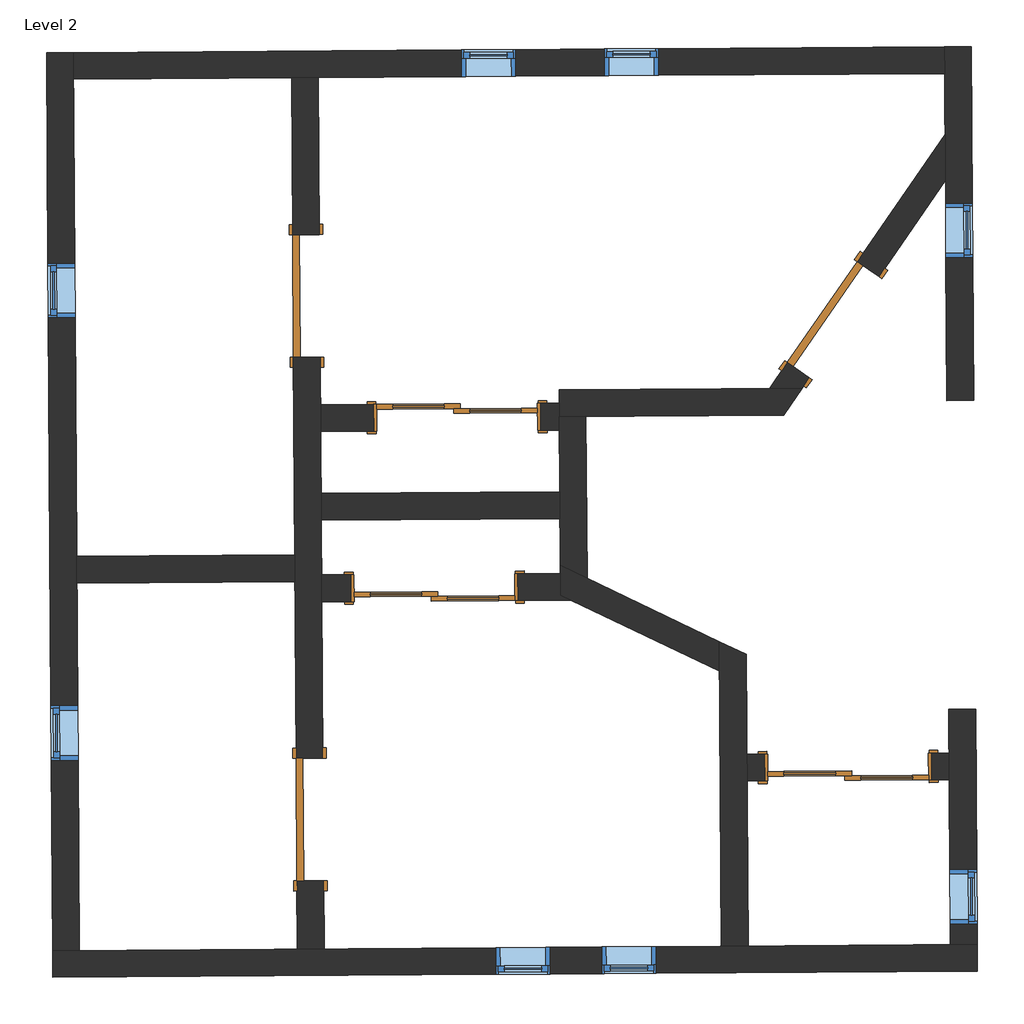
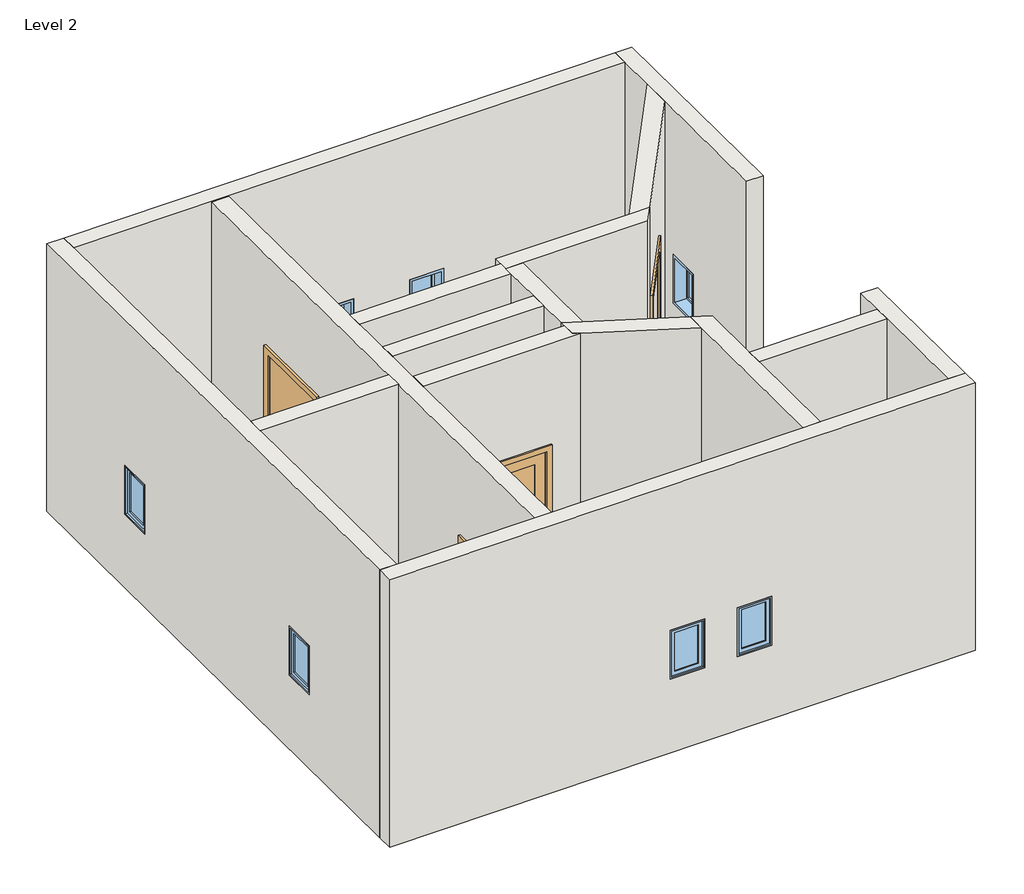
# One storey: 16 walls, 8 windows, 6 doors.
"""IFC4 building model written with IfcOpenShell, lengths in millimetres."""

import ifcopenshell
import ifcopenshell.guid

model = None  # the IFC model being written
_history = None  # IfcOwnerHistory: only IFC2X3 demands one
_inside = {}  # id of a spatial element -> (the spatial element, [elements in it])
_under = {}  # id of a project, library or spatial element -> (it, [spatial elements below it])
_declared = {}  # id of a project -> (the project, [libraries it declares])
_typed = {}  # id of a type object -> (the type object, [elements of that type])
_made_of = {}  # id of a material, layer set ... -> (it, [elements and type objects made of it])


def new_model(schema):
    """Start an empty IFC model of exactly this schema.

    Asked for "IFC4X3", IfcOpenShell would pick the latest addendum, in which some entities
    have other attributes; the version numbers below select the first issue.
    IFC2X3 requires an IfcOwnerHistory on every rooted entity: one is made here for all.
    """
    global model, _history
    if schema == "IFC4X3":
        model = ifcopenshell.file(schema_version=(4, 3, 0, 0))
    else:
        model = ifcopenshell.file(schema=schema)
    _inside.clear()
    _under.clear()
    _declared.clear()
    _typed.clear()
    _made_of.clear()
    _history = None
    if model.schema == "IFC2X3":
        org = make("IfcOrganization", Name="unknown")
        user = make(
            "IfcPersonAndOrganization",
            ThePerson=make("IfcPerson", FamilyName="unknown"),
            TheOrganization=org,
        )
        app = make(
            "IfcApplication",
            ApplicationDeveloper=org,
            Version="unknown",
            ApplicationFullName="unknown",
            ApplicationIdentifier="unknown",
        )
        _history = make(
            "IfcOwnerHistory",
            OwningUser=user,
            OwningApplication=app,
            ChangeAction="ADDED",
            CreationDate=0,
        )
    return model


def make(cls, **values):
    """One entity of the class cls with the attributes given. An attribute that is None is left unset."""
    return model.create_entity(
        cls, **{name: value for name, value in values.items() if value is not None}
    )


def rooted(cls, **values):
    """An entity with a GlobalId (a new one), such as an element, a storey or a relation."""
    return make(cls, GlobalId=ifcopenshell.guid.new(), OwnerHistory=_history, **values)


def si_unit(unit_type, name, prefix=None):
    """IfcSIUnit, for example si_unit("LENGTHUNIT", "METRE", prefix="MILLI")."""
    return make("IfcSIUnit", UnitType=unit_type, Prefix=prefix, Name=name)


def assignment(units):
    """IfcUnitAssignment: the units of a project."""
    return None if units is None else make("IfcUnitAssignment", Units=units)


def point(xyz):
    """IfcCartesianPoint."""
    return None if xyz is None else make("IfcCartesianPoint", Coordinates=xyz)


def direction(xyz):
    """IfcDirection."""
    return None if xyz is None else make("IfcDirection", DirectionRatios=xyz)


def frame(location, z_axis=None, x_axis=None):
    """IfcAxis2Placement3D, a coordinate frame: its origin and axes. An axis left out is left unset."""
    return make(
        "IfcAxis2Placement3D",
        Location=point(location),
        Axis=direction(z_axis),
        RefDirection=direction(x_axis),
    )


def origin():
    """The frame at (0, 0, 0) with its axes left unset."""
    return frame((0.0, 0.0, 0.0))


def origin_with_axes():
    """The frame at (0, 0, 0) with the z axis (0, 0, 1) and the x axis (1, 0, 0) written out."""
    return frame((0.0, 0.0, 0.0), z_axis=(0.0, 0.0, 1.0), x_axis=(1.0, 0.0, 0.0))


def place(relative_to, where):
    """IfcLocalPlacement: puts the frame where relative to a parent placement (None: the world)."""
    return make(
        "IfcLocalPlacement", PlacementRelTo=relative_to, RelativePlacement=where
    )


def context(
    kind, dimensions, precision=None, world=None, true_north=None, identifier=None
):
    """IfcGeometricRepresentationContext, for example the 3D "Model" context."""
    return make(
        "IfcGeometricRepresentationContext",
        ContextIdentifier=identifier,
        ContextType=kind,
        CoordinateSpaceDimension=dimensions,
        Precision=precision,
        WorldCoordinateSystem=world,
        TrueNorth=true_north,
    )


def project(units=None, contexts=None):
    """IfcProject with its units and contexts."""
    return rooted(
        "IfcProject",
        Name="project",
        RepresentationContexts=contexts,
        UnitsInContext=assignment(units),
    )


def spatial(cls, under=None, at=None, **own):
    """A site, building, storey or space (cls), placed at a placement, below another one or the project."""
    s = rooted(cls, ObjectPlacement=at, **own)
    if under is not None:
        _under.setdefault(under.id(), (under, []))[1].append(s)
    return s


def polyline(points):
    """IfcPolyline through the points."""
    return make("IfcPolyline", Points=[point(p) for p in points])


def outline(outer, holes=None, kind="AREA"):
    """IfcArbitraryClosedProfileDef: a profile drawn as a closed curve; with holes, ...WithVoids."""
    if holes is None:
        return make("IfcArbitraryClosedProfileDef", ProfileType=kind, OuterCurve=outer)
    return make(
        "IfcArbitraryProfileDefWithVoids",
        ProfileType=kind,
        OuterCurve=outer,
        InnerCurves=holes,
    )


def extrude(swept, where, along, depth):
    """IfcExtrudedAreaSolid: the profile swept, set in the frame where, extruded along a direction by depth."""
    return make(
        "IfcExtrudedAreaSolid",
        SweptArea=swept,
        Position=where,
        ExtrudedDirection=direction(along),
        Depth=depth,
    )


def faces_of(points, faces, orient=None, outer=None):
    """IfcFace entities. A face is a list of loops; a loop is a list of indices into points, from 0.

    orient and outer hold one flag for each loop. By default every Orientation is true, the
    first loop of a face is its IfcFaceOuterBound and the others are IfcFaceBound.
    """
    made = []
    for i, loops in enumerate(faces):
        bounds = []
        for j, loop in enumerate(loops):
            is_outer = j == 0 if outer is None else outer[i][j]
            bounds.append(
                make(
                    "IfcFaceOuterBound" if is_outer else "IfcFaceBound",
                    Bound=make("IfcPolyLoop", Polygon=[points[k] for k in loop]),
                    Orientation=True if orient is None else orient[i][j],
                )
            )
        made.append(make("IfcFace", Bounds=bounds))
    return made


def faceted_brep(points, faces, orient=None, outer=None, voids=None):
    """IfcFacetedBrep: a solid bounded by flat faces; with voids (closed shells), ...WithVoids."""
    shared = [point(p) for p in points]
    hull = make("IfcClosedShell", CfsFaces=faces_of(shared, faces, orient, outer))
    if voids is None:
        return make("IfcFacetedBrep", Outer=hull)
    return make(
        "IfcFacetedBrepWithVoids",
        Outer=hull,
        Voids=[
            make(cls, CfsFaces=faces_of(shared, fs, o, b)) for cls, fs, o, b in voids
        ],
    )


def shape(context_of_items, identifier, shape_type, items):
    """IfcShapeRepresentation: the items that make up one representation, for example the "Body"."""
    return make(
        "IfcShapeRepresentation",
        ContextOfItems=context_of_items,
        RepresentationIdentifier=identifier,
        RepresentationType=shape_type,
        Items=items,
    )


def source(mapping_origin, context_of_items, identifier, shape_type, items):
    """IfcRepresentationMap: a shape defined once, which mapped items show again and again."""
    return make(
        "IfcRepresentationMap",
        MappingOrigin=mapping_origin,
        MappedRepresentation=shape(context_of_items, identifier, shape_type, items),
    )


def transform(
    local_origin,
    x_axis=None,
    y_axis=None,
    z_axis=None,
    scale=None,
    scale2=None,
    scale3=None,
    uniform=True,
):
    """IfcCartesianTransformationOperator3D, or its non-uniform kind. x_axis, y_axis, z_axis: its Axis1, 2, 3."""
    if uniform:
        return make(
            "IfcCartesianTransformationOperator3D",
            Axis1=direction(x_axis),
            Axis2=direction(y_axis),
            LocalOrigin=point(local_origin),
            Scale=scale,
            Axis3=direction(z_axis),
        )
    return make(
        "IfcCartesianTransformationOperator3DnonUniform",
        Axis1=direction(x_axis),
        Axis2=direction(y_axis),
        LocalOrigin=point(local_origin),
        Scale=scale,
        Axis3=direction(z_axis),
        Scale2=scale2,
        Scale3=scale3,
    )


def mapped(mapping_source, mapping_target):
    """IfcMappedItem: shows the shape of a source again, moved by a transform."""
    return make(
        "IfcMappedItem", MappingSource=mapping_source, MappingTarget=mapping_target
    )


def made_of(thing, what):
    """Note that an element or type object is made of a material, layer set ...; save() writes the relation."""
    if what is not None:
        _made_of.setdefault(what.id(), (what, []))[1].append(thing)
    return thing


def element(
    cls,
    number,
    at=None,
    inside=None,
    cuts=None,
    type_object=None,
    material=None,
    context=None,
    identifier="Body",
    shape_type=None,
    held_by="IfcProductDefinitionShape",
    body=None,
    shapes=None,
    **own,
):
    """One element of the class cls, such as IfcWall. Its Tag is "e" and its number.

    at: its placement. inside: the storey or other place that contains it. cuts: it is an
    opening in that element (IfcRelVoidsElement). A single representation is given by context,
    identifier, shape_type and body (its items); several are given by shapes. held_by: the class
    of the entity that holds the representations. save() writes the other relations.
    """
    e = rooted(cls, Tag="e%d" % number, ObjectPlacement=at, **own)
    if body is not None:
        shapes = [shape(context, identifier, shape_type, body)]
    if shapes is not None:
        e.Representation = make(held_by, Representations=shapes)
    if inside is not None:
        _inside.setdefault(inside.id(), (inside, []))[1].append(e)
    if cuts is not None:
        rooted(
            "IfcRelVoidsElement", RelatingBuildingElement=cuts, RelatedOpeningElement=e
        )
    if type_object is not None:
        _typed.setdefault(type_object.id(), (type_object, []))[1].append(e)
    return made_of(e, material)


def aggregate(whole, parts):
    """IfcRelAggregates: a whole, such as a stair, and the parts it consists of."""
    return rooted("IfcRelAggregates", RelatingObject=whole, RelatedObjects=parts)


def save(model, path):
    """Write the relations noted so far, then the file.

    IfcRelAggregates (storeys below a building ...), IfcRelContainedInSpatialStructure (elements
    in a storey), IfcRelDefinesByType, IfcRelAssociatesMaterial and IfcRelDeclares: one each for
    every whole, place, type object, material and project.
    """
    for whole, parts in _under.values():
        aggregate(whole, parts)
    for where, things in _inside.values():
        rooted(
            "IfcRelContainedInSpatialStructure",
            RelatedElements=things,
            RelatingStructure=where,
        )
    for kind, things in _typed.values():
        rooted("IfcRelDefinesByType", RelatedObjects=things, RelatingType=kind)
    for what, things in _made_of.values():
        rooted("IfcRelAssociatesMaterial", RelatedObjects=things, RelatingMaterial=what)
    for by, libraries in _declared.values():
        rooted("IfcRelDeclares", RelatingContext=by, RelatedDefinitions=libraries)
    model.write(path)


def m_door_interior_double_sliding_2_panel_wood_1200_x_2000mm_2523b4d6(model_context):
    return source(origin(), model_context, "Body", "SweptSolid", [
        extrude(outline(polyline([(480.0, 38.4916667), (94.6, 38.4916667), (94.6, 50.1583333), (480.0, 50.1583333), (480.0, 38.4916667)])), frame((0.0, 0.0, 1014.4), z_axis=(0.0, 0.0, 1.0), x_axis=(1.0, 0.0, 0.0)), (0.0, 0.0, 1.0), 865.6),
        extrude(outline(polyline([(480.0, 38.4916667), (94.6, 38.4916667), (94.6, 50.1583333), (480.0, 50.1583333), (480.0, 38.4916667)])), frame((0.0, 0.0, 230.0), z_axis=(0.0, 0.0, 1.0), x_axis=(1.0, 0.0, 0.0)), (0.0, 0.0, 1.0), 584.4),
        extrude(outline(polyline([(2000.0, -25.4), (0.0, -25.4), (0.0, 600.0), (2000.0, 600.0), (2000.0, -25.4)]), holes=[polyline([(1880.0, 94.6), (1880.0, 480.0), (1014.4, 480.0), (1014.4, 94.6), (1880.0, 94.6)]), polyline([(814.4, 94.6), (814.4, 480.0), (230.0, 480.0), (230.0, 94.6), (814.4, 94.6)])]), frame((0.0, 26.825, 0.0), z_axis=(0.0, 1.0, 0.0), x_axis=(0.0, 0.0, 1.0)), (0.0, 0.0, 1.0), 35.0),
        extrude(outline(polyline([(-94.6, 73.4916667), (-480.0, 73.4916667), (-480.0, 85.1583333), (-94.6, 85.1583333), (-94.6, 73.4916667)])), frame((0.0, 0.0, 1014.4), z_axis=(0.0, 0.0, 1.0), x_axis=(1.0, 0.0, 0.0)), (0.0, 0.0, 1.0), 865.6),
        extrude(outline(polyline([(-94.6, 73.4916667), (-480.0, 73.4916667), (-480.0, 85.1583333), (-94.6, 85.1583333), (-94.6, 73.4916667)])), frame((0.0, 0.0, 230.0), z_axis=(0.0, 0.0, 1.0), x_axis=(1.0, 0.0, 0.0)), (0.0, 0.0, 1.0), 584.4),
        extrude(outline(polyline([(2000.0, -600.0), (0.0, -600.0), (0.0, 25.4), (2000.0, 25.4), (2000.0, -600.0)]), holes=[polyline([(1880.0, -480.0), (1880.0, -94.6), (1014.4, -94.6), (1014.4, -480.0), (1880.0, -480.0)]), polyline([(814.4, -480.0), (814.4, -94.6), (230.0, -94.6), (230.0, -480.0), (814.4, -480.0)])]), frame((0.0, 61.825, 0.0), z_axis=(0.0, 1.0, 0.0), x_axis=(0.0, 0.0, 1.0)), (0.0, 0.0, 1.0), 35.0),
        extrude(outline(polyline([(0.0, 600.0), (0.0, 625.0), (2025.0, 625.0), (2025.0, -625.0), (0.0, -625.0), (0.0, -600.0), (2000.0, -600.0), (2000.0, 600.0), (0.0, 600.0)])), frame((0.0, -103.175, 0.0), z_axis=(0.0, 1.0, 0.0), x_axis=(0.0, 0.0, 1.0)), (0.0, 0.0, 1.0), 200.0),
        extrude(outline(polyline([(0.0, 606.35), (0.0, 671.35), (2071.35, 671.35), (2071.35, -671.35), (0.0, -671.35), (0.0, -606.35), (2006.35, -606.35), (2006.35, 606.35), (0.0, 606.35)])), frame((0.0, -123.175, 0.0), z_axis=(0.0, 1.0, 0.0), x_axis=(0.0, 0.0, 1.0)), (0.0, 0.0, 1.0), 20.0),
        extrude(outline(polyline([(0.0, 606.35), (0.0, 671.35), (2071.35, 671.35), (2071.35, -671.35), (0.0, -671.35), (0.0, -606.35), (2006.35, -606.35), (2006.35, 606.35), (0.0, 606.35)])), frame((0.0, 96.825, 0.0), z_axis=(0.0, 1.0, 0.0), x_axis=(0.0, 0.0, 1.0)), (0.0, 0.0, 1.0), 20.0),
    ])


def m_single_flush_0915_x_2134mm_6a9e8738(model_context):
    return source(origin(), model_context, "Body", "SweptSolid", [
        extrude(outline(polyline([(2210.0, -533.5), (0.0, -533.5), (0.0, -457.5), (2134.0, -457.5), (2134.0, 457.5), (0.0, 457.5), (0.0, 533.5), (2210.0, 533.5), (2210.0, -533.5)])), frame((0.0, 100.0, 0.0), z_axis=(0.0, 1.0, 0.0), x_axis=(0.0, 0.0, 1.0)), (0.0, 0.0, 1.0), 25.0),
        extrude(outline(polyline([(2210.0, 533.5), (2210.0, -533.5), (0.0, -533.5), (0.0, -457.5), (2134.0, -457.5), (2134.0, 457.5), (0.0, 457.5), (0.0, 533.5), (2210.0, 533.5)])), frame((0.0, -125.0, 0.0), z_axis=(0.0, 1.0, 0.0), x_axis=(0.0, 0.0, 1.0)), (0.0, 0.0, 1.0), 25.0),
        extrude(outline(polyline([(457.5, 49.0), (-457.5, 49.0), (-457.5, 100.0), (457.5, 100.0), (457.5, 49.0)])), origin_with_axes(), (0.0, 0.0, 1.0), 2134.0),
    ])


def m_single_flush_0915_x_2134mm_727434cd(model_context):
    return source(origin(), model_context, "Body", "SweptSolid", [
        extrude(outline(polyline([(2210.0, -533.5), (0.0, -533.5), (0.0, -457.5), (2134.0, -457.5), (2134.0, 457.5), (0.0, 457.5), (0.0, 533.5), (2210.0, 533.5), (2210.0, -533.5)])), frame((0.0, -125.0, 0.0), z_axis=(0.0, 1.0, 0.0), x_axis=(0.0, 0.0, 1.0)), (0.0, 0.0, 1.0), 25.0),
        extrude(outline(polyline([(2210.0, 533.5), (2210.0, -533.5), (0.0, -533.5), (0.0, -457.5), (2134.0, -457.5), (2134.0, 457.5), (0.0, 457.5), (0.0, 533.5), (2210.0, 533.5)])), frame((0.0, 100.0, 0.0), z_axis=(0.0, 1.0, 0.0), x_axis=(0.0, 0.0, 1.0)), (0.0, 0.0, 1.0), 25.0),
        extrude(outline(polyline([(457.5, -49.0), (457.5, -100.0), (-457.5, -100.0), (-457.5, -49.0), (457.5, -49.0)])), origin_with_axes(), (0.0, 0.0, 1.0), 2134.0),
    ])


def m_fixed_0406_x_0610mm_8205b201(model_context):
    return source(origin(), model_context, "Body", "SweptSolid", [
        extrude(outline(polyline([(-140.0, 78.0), (140.0, 78.0), (140.0, 66.0), (-140.0, 66.0), (-140.0, 78.0)])), frame((0.0, 0.0, 978.0), z_axis=(0.0, 0.0, 1.0), x_axis=(1.0, 0.0, 0.0)), (0.0, 0.0, 1.0), 484.0),
        extrude(outline(polyline([(1506.0, -184.0), (934.0, -184.0), (934.0, 184.0), (1506.0, 184.0), (1506.0, -184.0)]), holes=[polyline([(1462.0, -140.0), (1462.0, 140.0), (978.0, 140.0), (978.0, -140.0), (1462.0, -140.0)])]), frame((0.0, 50.0, 0.0), z_axis=(0.0, 1.0, 0.0), x_axis=(0.0, 0.0, 1.0)), (0.0, 0.0, 1.0), 44.0),
        extrude(outline(polyline([(1525.0, -203.0), (915.0, -203.0), (915.0, 203.0), (1525.0, 203.0), (1525.0, -203.0)]), holes=[polyline([(1506.0, -184.0), (1506.0, 184.0), (934.0, 184.0), (934.0, -184.0), (1506.0, -184.0)])]), frame((0.0, 50.0, 0.0), z_axis=(0.0, 1.0, 0.0), x_axis=(0.0, 0.0, 1.0)), (0.0, 0.0, 1.0), 63.0),
        extrude(outline(polyline([(1525.0, -203.0), (915.0, -203.0), (915.0, 203.0), (1525.0, 203.0), (1525.0, -203.0)]), holes=[polyline([(1493.0, -171.0), (1493.0, 171.0), (947.0, 171.0), (947.0, -171.0), (1493.0, -171.0)])]), frame((0.0, -87.0, 0.0), z_axis=(0.0, 1.0, 0.0), x_axis=(0.0, 0.0, 1.0)), (0.0, 0.0, 1.0), 137.0),
    ])


model = new_model("IFC4")

# Units and contexts
model_context = context("Model", 3, world=origin())
ifc_project = project(units=[si_unit("LENGTHUNIT", "METRE", prefix="MILLI")], contexts=[model_context])

# Site, building, storey
site = spatial("IfcSite", under=ifc_project)
building = spatial("IfcBuilding", under=site)
storey = spatial("IfcBuildingStorey", under=building, Name="Level 2", Elevation=3048.0)

# Doors
placement = place(None, origin())
m_door_interior_double_sliding_2_panel_wood_1200_x_2000mm_shape = m_door_interior_double_sliding_2_panel_wood_1200_x_2000mm_2523b4d6(model_context)
element("IfcDoor", 1, ObjectType="M_Door-Interior-Double-Sliding-2_Panel-Wood : 1200 x 2000mm", at=placement, inside=storey, context=model_context, shape_type="MappedRepresentation", body=[
    mapped(m_door_interior_double_sliding_2_panel_wood_1200_x_2000mm_shape, transform((-90488.9924739, -37950.707077, 3048.0), x_axis=(0.9999777944135733, 0.006664133834601911, 0.0), y_axis=(-0.006664133834601911, 0.9999777944135733, 0.0), z_axis=(0.0, 0.0, 1.0))),
])
element("IfcDoor", 2, ObjectType="M_Door-Interior-Double-Sliding-2_Panel-Wood : 1200 x 2000mm", at=placement, inside=storey, context=model_context, shape_type="MappedRepresentation", body=[
    mapped(m_door_interior_double_sliding_2_panel_wood_1200_x_2000mm_shape, transform((-90659.0777486, -39228.968042, 3048.0), x_axis=(-0.9999777944135733, -0.006664133834601911, 0.0), y_axis=(0.006664133834601911, -0.9999777944135733, 0.0), z_axis=(0.0, 0.0, 1.0))),
])
element("IfcDoor", 3, ObjectType="M_Door-Interior-Double-Sliding-2_Panel-Wood : 1200 x 2000mm", at=placement, inside=storey, context=model_context, shape_type="MappedRepresentation", body=[
    mapped(m_door_interior_double_sliding_2_panel_wood_1200_x_2000mm_shape, transform((-87568.9864205, -40568.3479238, 3048.0), x_axis=(-0.9999777944135733, -0.006664133834601911, 0.0), y_axis=(0.006664133834601911, -0.9999777944135733, 0.0), z_axis=(0.0, 0.0, 1.0))),
])
m_single_flush_0915_x_2134mm_shape = m_single_flush_0915_x_2134mm_6a9e8738(model_context)
element("IfcDoor", 4, ObjectType="M_Single-Flush : 0915 x 2134mm", at=placement, inside=storey, context=model_context, shape_type="MappedRepresentation", body=[
    mapped(m_single_flush_0915_x_2134mm_shape, transform((-87680.4573367, -37224.8879698, 3048.0), x_axis=(0.5681047608958888, 0.8229562446736918, 0.0), y_axis=(-0.8229562446736918, 0.5681047608958888, 0.0), z_axis=(0.0, 0.0, 1.0))),
])
element("IfcDoor", 5, ObjectType="M_Single-Flush : 0915 x 2134mm", at=placement, inside=storey, context=model_context, shape_type="MappedRepresentation", body=[
    mapped(m_single_flush_0915_x_2134mm_shape, transform((-91614.2394972, -37047.0582792, 3048.0), x_axis=(-0.0066641338345986775, 0.9999777944135734, 0.0), y_axis=(-0.9999777944135734, -0.0066641338345986775, 0.0), z_axis=(0.0, 0.0, 1.0))),
])
m_single_flush_0915_x_2134mm_2_shape = m_single_flush_0915_x_2134mm_727434cd(model_context)
element("IfcDoor", 6, ObjectType="M_Single-Flush : 0915 x 2134mm", at=placement, inside=storey, context=model_context, shape_type="MappedRepresentation", body=[
    mapped(m_single_flush_0915_x_2134mm_2_shape, transform((-91588.1820843, -40957.0689247, 3048.0), x_axis=(0.0066641338345986775, -0.9999777944135734, 0.0), y_axis=(0.9999777944135734, 0.0066641338345986775, 0.0), z_axis=(0.0, 0.0, 1.0))),
])

# Walls
element("IfcWall", 7, ObjectType="Generic - 200mm", at=placement, inside=storey, context=model_context, shape_type="Brep", body=[
    faceted_brep([(-86605.0497125, -41890.681395, 3048.0), (-86805.0452714, -41892.0142218, 3048.0), (-88315.2179284, -41902.078438, 3048.0), (-88515.2134873, -41903.4112648, 3048.0), (-91481.7414203, -41923.1810429, 3048.0), (-91681.7369792, -41924.5138697, 3048.0), (-93310.5008107, -41935.3684109, 3048.0), (-93510.4963696, -41936.7012377, 3048.0), (-93510.4963696, -41936.7012377, 6372.225), (-93310.5008107, -41935.3684109, 6372.225), (-88515.2134873, -41903.4112648, 6372.225), (-88315.2179284, -41902.078438, 6372.225), (-86805.0452714, -41892.0142218, 6372.225), (-86605.0497125, -41890.681395, 6372.225), (-89795.4819615, -41911.9433347, 3963.0), (-89795.4819615, -41911.9433347, 4573.0), (-90201.4729461, -41914.648973, 4573.0), (-90201.4729461, -41914.648973, 3963.0), (-89003.8510886, -41906.6676834, 3963.0), (-89003.8510886, -41906.6676834, 4573.0), (-89409.8420731, -41909.3733218, 4573.0), (-89409.8420731, -41909.3733218, 3963.0), (-86603.7168857, -42090.6769539, 3048.0), (-86603.7168857, -42090.6769539, 6372.225), (-93509.1635428, -42136.6967965, 6372.225), (-93509.1635428, -42136.6967965, 3048.0), (-89794.1491348, -42111.9388936, 3963.0), (-90200.1401193, -42114.6445319, 3963.0), (-90200.1401193, -42114.6445319, 4573.0), (-89794.1491348, -42111.9388936, 4573.0), (-89002.5182618, -42106.6632423, 3963.0), (-89408.5092463, -42109.3688807, 3963.0), (-89408.5092463, -42109.3688807, 4573.0), (-89002.5182618, -42106.6632423, 4573.0)], [[[0, 1, 2, 3, 4, 5, 6, 7, 8, 9, 10, 11, 12, 13], [14, 15, 16, 17], [18, 19, 20, 21]], [[22, 23, 24, 25], [26, 27, 28, 29], [30, 31, 32, 33]], [[8, 7, 25, 24]], [[0, 13, 23, 22]], [[15, 14, 26, 29]], [[16, 15, 29, 28]], [[17, 16, 28, 27]], [[14, 17, 27, 26]], [[19, 18, 30, 33]], [[20, 19, 33, 32]], [[21, 20, 32, 31]], [[18, 21, 31, 30]], [[7, 6, 5, 4, 3, 2, 1, 0, 22, 25]], [[13, 12, 11, 10, 9, 8, 24, 23]]]),
])
element("IfcWall", 8, ObjectType="Generic - 200mm", at=placement, inside=storey, context=model_context, shape_type="Brep", body=[
    faceted_brep([(-93310.5008107, -41935.3684109, 3048.0), (-93328.7831618, -39192.0343866, 3048.0), (-93330.1159886, -38992.0388277, 3048.0), (-93353.8549998, -35429.9128716, 3048.0), (-93355.1878266, -35229.9173127, 3048.0), (-93355.1878266, -35229.9173127, 6372.225), (-93353.8549998, -35429.9128716, 6372.225), (-93330.1159886, -38992.0388277, 6372.225), (-93328.7831618, -39192.0343866, 6372.225), (-93310.5008107, -41935.3684109, 6372.225), (-93341.9968401, -37209.2733589, 3963.0), (-93341.9968401, -37209.2733589, 4573.0), (-93344.7024784, -36803.2823744, 4573.0), (-93344.7024784, -36803.2823744, 3963.0), (-93319.971844, -40514.2050264, 3963.0), (-93319.971844, -40514.2050264, 4573.0), (-93322.6774824, -40108.2140418, 4573.0), (-93322.6774824, -40108.2140418, 3963.0), (-93510.4963696, -41936.7012377, 3048.0), (-93510.4963696, -41936.7012377, 6372.225), (-93555.1833855, -35231.2501394, 6372.225), (-93555.1833855, -35231.2501394, 3048.0), (-93541.9923989, -37210.6061857, 3963.0), (-93544.6980373, -36804.6152012, 3963.0), (-93544.6980373, -36804.6152012, 4573.0), (-93541.9923989, -37210.6061857, 4573.0), (-93519.9674029, -40515.5378531, 3963.0), (-93522.6730413, -40109.5468686, 3963.0), (-93522.6730413, -40109.5468686, 4573.0), (-93519.9674029, -40515.5378531, 4573.0)], [[[0, 1, 2, 3, 4, 5, 6, 7, 8, 9], [10, 11, 12, 13], [14, 15, 16, 17]], [[18, 19, 20, 21], [22, 23, 24, 25], [26, 27, 28, 29]], [[4, 3, 2, 1, 0, 18, 21]], [[9, 8, 7, 6, 5, 20, 19]], [[0, 9, 19, 18]], [[5, 4, 21, 20]], [[11, 10, 22, 25]], [[12, 11, 25, 24]], [[13, 12, 24, 23]], [[10, 13, 23, 22]], [[15, 14, 26, 29]], [[16, 15, 29, 28]], [[17, 16, 28, 27]], [[14, 17, 27, 26]]]),
])
element("IfcWall", 9, ObjectType="Generic - 200mm", at=placement, inside=storey, context=model_context, shape_type="Brep", body=[
    faceted_brep([(-93353.8549998, -35429.9128716, 3048.0), (-91725.0911683, -35419.0583304, 3048.0), (-91525.0956094, -35417.7255036, 3048.0), (-86848.3994605, -35386.5586825, 3048.0), (-86848.3994605, -35386.5586825, 6372.225), (-93353.8549998, -35429.9128716, 6372.225), (-89389.7430272, -35403.4949122, 3963.0), (-89389.7430272, -35403.4949122, 4573.0), (-88983.7520427, -35400.7892739, 4573.0), (-88983.7520427, -35400.7892739, 3963.0), (-90456.5193383, -35410.6042102, 3963.0), (-90456.5193383, -35410.6042102, 4573.0), (-90050.5283537, -35407.8985718, 4573.0), (-90050.5283537, -35407.8985718, 3963.0), (-93355.1878266, -35229.9173127, 3048.0), (-93355.1878266, -35229.9173127, 6372.225), (-86849.7322872, -35186.5631236, 6372.225), (-86849.7322872, -35186.5631236, 3048.0), (-89391.075854, -35203.4993533, 3963.0), (-88985.0848694, -35200.793715, 3963.0), (-88985.0848694, -35200.793715, 4573.0), (-89391.075854, -35203.4993533, 4573.0), (-90457.852165, -35210.6086513, 3963.0), (-90051.8611805, -35207.903013, 3963.0), (-90051.8611805, -35207.903013, 4573.0), (-90457.852165, -35210.6086513, 4573.0)], [[[0, 1, 2, 3, 4, 5], [6, 7, 8, 9], [10, 11, 12, 13]], [[14, 15, 16, 17], [18, 19, 20, 21], [22, 23, 24, 25]], [[3, 2, 1, 0, 14, 17]], [[5, 4, 16, 15]], [[0, 5, 15, 14]], [[7, 6, 18, 21]], [[8, 7, 21, 20]], [[9, 8, 20, 19]], [[6, 9, 19, 18]], [[11, 10, 22, 25]], [[12, 11, 25, 24]], [[13, 12, 24, 23]], [[10, 13, 23, 22]], [[4, 3, 17, 16]]]),
])
element("IfcWall", 10, ObjectType="Generic - 200mm", at=placement, inside=storey, context=model_context, shape_type="Brep", body=[
    faceted_brep([(-86849.7322872, -35186.5631236, 3048.0), (-86848.3994605, -35386.5586825, 3048.0), (-86845.3830911, -35839.1760037, 3048.0), (-86843.0593785, -36187.85762, 3048.0), (-86832.1189478, -37829.5094911, 3048.0), (-86832.1189478, -37829.5094911, 6372.225), (-86843.0593785, -36187.85762, 6372.225), (-86845.3830911, -35839.1760037, 6372.225), (-86848.3994605, -35386.5586825, 6372.225), (-86849.7322872, -35186.5631236, 6372.225), (-86841.94523, -36355.0397048, 3963.0), (-86841.94523, -36355.0397048, 4573.0), (-86839.2395917, -36761.0306894, 4573.0), (-86839.2395917, -36761.0306894, 3963.0), (-86649.7367284, -35185.2302968, 3048.0), (-86649.7367284, -35185.2302968, 6372.225), (-86632.1233889, -37828.1766644, 6372.225), (-86632.1233889, -37828.1766644, 3048.0), (-86641.9496711, -36353.7068781, 3963.0), (-86639.2440328, -36759.6978626, 3963.0), (-86639.2440328, -36759.6978626, 4573.0), (-86641.9496711, -36353.7068781, 4573.0)], [[[0, 1, 2, 3, 4, 5, 6, 7, 8, 9], [10, 11, 12, 13]], [[14, 15, 16, 17], [18, 19, 20, 21]], [[4, 3, 2, 1, 0, 14, 17]], [[5, 4, 17, 16]], [[9, 8, 7, 6, 5, 16, 15]], [[11, 10, 18, 21]], [[12, 11, 21, 20]], [[13, 12, 20, 19]], [[10, 13, 19, 18]], [[0, 9, 15, 14]]]),
])
element("IfcWall", 11, ObjectType="Generic - 200mm", at=placement, inside=storey, context=model_context, shape_type="Brep", body=[
    faceted_brep([(-86605.0497125, -41890.681395, 3048.0), (-86616.7572548, -40133.9216051, 3048.0), (-86616.7572548, -40133.9216051, 6372.225), (-86605.0497125, -41890.681395, 6372.225), (-86608.7829603, -41330.4938346, 3963.0), (-86606.077322, -41736.4848191, 3963.0), (-86606.077322, -41736.4848191, 4573.0), (-86608.7829603, -41330.4938346, 4573.0), (-86805.0452714, -41892.0142218, 3048.0), (-86805.0452714, -41892.0142218, 6372.225), (-86813.2548373, -40660.1386656, 6372.225), (-86814.587664, -40460.1431068, 6372.225), (-86816.7528137, -40135.2544319, 6372.225), (-86816.7528137, -40135.2544319, 3048.0), (-86814.587664, -40460.1431068, 3048.0), (-86813.2548373, -40660.1386656, 3048.0), (-86808.7785192, -41331.8266614, 3963.0), (-86808.7785192, -41331.8266614, 4573.0), (-86806.0728808, -41737.8176459, 4573.0), (-86806.0728808, -41737.8176459, 3963.0)], [[[0, 1, 2, 3], [4, 5, 6, 7]], [[8, 9, 10, 11, 12, 13, 14, 15], [16, 17, 18, 19]], [[1, 0, 8, 15, 14, 13]], [[2, 1, 13, 12]], [[3, 2, 12, 11, 10, 9]], [[0, 3, 9, 8]], [[17, 16, 4, 7]], [[18, 17, 7, 6]], [[19, 18, 6, 5]], [[16, 19, 5, 4]]]),
])
element("IfcWall", 12, ObjectType="Generic - 200mm", at=placement, inside=storey, context=model_context, shape_type="Brep", body=[
    faceted_brep([(-91685.1310226, -41415.225179, 5182.0), (-91685.1310226, -41415.225179, 3048.0), (-91681.7369792, -41924.5138697, 3048.0), (-91681.7369792, -41924.5138697, 6363.9898437), (-91725.0911683, -35419.0583304, 6363.9898437), (-91725.0911683, -35419.0583304, 3048.0), (-91717.2861179, -36590.2348516, 3048.0), (-91717.2861179, -36590.2348516, 5182.0), (-91711.1884354, -37505.2145335, 5182.0), (-91711.1884354, -37505.2145335, 3048.0), (-91701.352157, -38981.1842865, 3048.0), (-91700.0193303, -39181.1798454, 3048.0), (-91691.228705, -40500.2454971, 3048.0), (-91691.228705, -40500.2454971, 5182.0), (-91481.7414203, -41923.1810429, 3048.0), (-91485.1354637, -41413.8923522, 3048.0), (-91485.1354637, -41413.8923522, 5182.0), (-91491.2331461, -40498.9126703, 5182.0), (-91491.2331461, -40498.9126703, 3048.0), (-91499.0138278, -39331.3927629, 3048.0), (-91500.3466546, -39131.397204, 3048.0), (-91503.0706134, -38722.657171, 3048.0), (-91504.4034401, -38522.6616122, 3048.0), (-91507.48227, -38060.6718711, 3048.0), (-91508.8150967, -37860.6763123, 3048.0), (-91511.1928765, -37503.8817068, 3048.0), (-91511.1928765, -37503.8817068, 5182.0), (-91517.290559, -36588.9020249, 5182.0), (-91517.290559, -36588.9020249, 3048.0), (-91525.0956094, -35417.7255036, 3048.0), (-91525.0956094, -35417.7255036, 6363.9898437), (-91481.7414203, -41923.1810429, 6363.9898437)], [[[0, 1, 2, 3, 4, 5, 6, 7, 8, 9, 10, 11, 12, 13]], [[14, 15, 16, 17, 18, 19, 20, 21, 22, 23, 24, 25, 26, 27, 28, 29, 30, 31]], [[3, 2, 14, 31]], [[5, 4, 30, 29]], [[7, 6, 28, 27]], [[8, 7, 27, 26]], [[9, 8, 26, 25]], [[16, 15, 1, 0]], [[17, 16, 0, 13]], [[18, 17, 13, 12]], [[29, 28, 6, 5]], [[2, 1, 15, 14]], [[12, 11, 10, 9, 25, 24, 23, 22, 21, 20, 19, 18]], [[4, 3, 31, 30]]]),
])
element("IfcWall", 13, ObjectType="Generic - 200mm", at=placement, inside=storey, context=model_context, shape_type="Brep", body=[
    faceted_brep([(-89726.9882359, -37948.8039365, 3048.0), (-89526.9926771, -37947.4711097, 3048.0), (-88050.9687487, -37937.6344703, 3048.0), (-88050.9687487, -37937.6344703, 6372.225), (-89526.9926771, -37947.4711097, 6372.225), (-89726.9882359, -37948.8039365, 6372.225), (-89728.3210627, -37748.8083776, 3048.0), (-89728.3210627, -37748.8083776, 6372.225), (-88156.4126737, -37738.3327371, 6372.225), (-87912.2631775, -37736.7056561, 6372.225), (-87912.2631775, -37736.7056561, 3048.0), (-88156.4126737, -37738.3327371, 3048.0), (-89727.6546493, -37848.8061571, 3048.0), (-89727.6546493, -37848.8061571, 6372.225)], [[[0, 1, 2, 3, 4, 5]], [[6, 7, 8, 9, 10, 11]], [[2, 1, 0, 12, 6, 11, 10]], [[5, 4, 3, 9, 8, 7, 13]], [[3, 2, 10, 9]], [[0, 5, 13, 7, 6, 12]]]),
])
element("IfcWall", 14, ObjectType="Generic - 200mm", at=placement, inside=storey, context=model_context, shape_type="Brep", body=[
    faceted_brep([(-87338.2537841, -36905.195964, 5182.0), (-87338.2537841, -36905.195964, 3048.0), (-86843.0593785, -36187.85762, 3048.0), (-86843.0593785, -36187.85762, 6372.225), (-87912.2631775, -37736.7056561, 6372.225), (-87912.2631775, -37736.7056561, 3048.0), (-87858.0696403, -37658.2009278, 3048.0), (-87858.0696403, -37658.2009278, 5182.0), (-86845.3830911, -35839.1760037, 3048.0), (-87502.845033, -36791.5750118, 3048.0), (-87502.845033, -36791.5750118, 5182.0), (-88022.6608893, -37544.5799757, 5182.0), (-88022.6608893, -37544.5799757, 3048.0), (-88156.4126737, -37738.3327371, 3048.0), (-88156.4126737, -37738.3327371, 6372.225), (-86845.3830911, -35839.1760037, 6372.225)], [[[0, 1, 2, 3, 4, 5, 6, 7]], [[8, 9, 10, 11, 12, 13, 14, 15]], [[6, 5, 13, 12]], [[2, 1, 9, 8]], [[4, 3, 15, 14]], [[5, 4, 14, 13]], [[3, 2, 8, 15]], [[10, 9, 1, 0]], [[11, 10, 0, 7]], [[12, 11, 7, 6]]]),
])
element("IfcWall", 15, ObjectType="Generic - 200mm", at=placement, inside=storey, context=model_context, shape_type="Brep", body=[
    faceted_brep([(-88530.374734, -39628.4104216, 3048.0), (-88528.8925721, -39850.8142698, 3048.0), (-88515.2134873, -41903.4112648, 3048.0), (-88515.2134873, -41903.4112648, 6372.225), (-88528.8925721, -39850.8142698, 6372.225), (-88530.374734, -39628.4104216, 6372.225), (-88329.7308105, -39724.3671015, 3048.0), (-88329.7308105, -39724.3671015, 6372.225), (-88324.760321, -40470.2073229, 6372.225), (-88323.4274943, -40670.2028818, 6372.225), (-88315.2179284, -41902.078438, 6372.225), (-88315.2179284, -41902.078438, 3048.0), (-88323.4274943, -40670.2028818, 3048.0), (-88324.760321, -40470.2073229, 3048.0)], [[[0, 1, 2, 3, 4, 5]], [[6, 7, 8, 9, 10, 11, 12, 13]], [[2, 1, 0, 6, 13, 12, 11]], [[5, 4, 3, 10, 9, 8, 7]], [[3, 2, 11, 10]], [[0, 5, 7, 6]]]),
])
element("IfcWall", 16, ObjectType="Generic - 200mm", at=placement, inside=storey, context=model_context, shape_type="Brep", body=[
    faceted_brep([(-89718.1028952, -39282.081999, 3048.0), (-89640.8876755, -39319.0096865, 3048.0), (-88528.8925721, -39850.8142698, 3048.0), (-88528.8925721, -39850.8142698, 6372.225), (-89640.8876755, -39319.0096865, 6372.225), (-89718.1028952, -39282.081999, 6372.225), (-89719.5850571, -39059.6781508, 3048.0), (-89719.5850571, -39059.6781508, 6372.225), (-89518.9411335, -39155.6348307, 6372.225), (-88530.374734, -39628.4104216, 6372.225), (-88530.374734, -39628.4104216, 3048.0), (-89518.9411335, -39155.6348307, 3048.0), (-89719.1862072, -39119.5270488, 3048.0), (-89719.1862072, -39119.5270488, 6372.225)], [[[0, 1, 2, 3, 4, 5]], [[6, 7, 8, 9, 10, 11]], [[2, 1, 0, 12, 6, 11, 10]], [[5, 4, 3, 9, 8, 7, 13]], [[3, 2, 10, 9]], [[0, 5, 13, 7, 6, 12]]]),
])
element("IfcWall", 17, ObjectType="Generic - 200mm", at=placement, inside=storey, context=model_context, shape_type="Brep", body=[
    faceted_brep([(-89726.9882359, -37948.8039365, 3048.0), (-89726.3218225, -38048.801716, 3048.0), (-89723.2429927, -38510.791457, 3048.0), (-89721.910166, -38710.7870159, 3048.0), (-89719.5850571, -39059.6781508, 3048.0), (-89719.5850571, -39059.6781508, 6372.225), (-89721.910166, -38710.7870159, 6372.225), (-89723.2429927, -38510.791457, 6372.225), (-89726.3218225, -38048.801716, 6372.225), (-89726.9882359, -37948.8039365, 6372.225), (-89526.9926771, -37947.4711097, 3048.0), (-89526.9926771, -37947.4711097, 6372.225), (-89518.9411335, -39155.6348307, 6372.225), (-89518.9411335, -39155.6348307, 3048.0)], [[[0, 1, 2, 3, 4, 5, 6, 7, 8, 9]], [[10, 11, 12, 13]], [[4, 3, 2, 1, 0, 10, 13]], [[9, 8, 7, 6, 5, 12, 11]], [[0, 9, 11, 10]], [[5, 4, 13, 12]]]),
])
element("IfcWall", 18, ObjectType="Generic - 200mm", at=placement, inside=storey, context=model_context, shape_type="SweptSolid", body=[
    extrude(outline(polyline([(-93330.1159886, -38992.0388277), (-91701.352157, -38981.1842865), (-91700.0193303, -39181.1798454), (-93328.7831618, -39192.0343866), (-93330.1159886, -38992.0388277)])), frame((0.0, 0.0, 3048.0), z_axis=(0.0, 0.0, 1.0), x_axis=(1.0, 0.0, 0.0)), (0.0, 0.0, 1.0), 3324.225),
])
element("IfcWall", 19, ObjectType="Generic - 200mm", at=placement, inside=storey, context=model_context, shape_type="Brep", body=[
    faceted_brep([(-91508.8150967, -37860.6763123, 6372.225), (-89727.6546493, -37848.8061571, 6372.225), (-89727.6546493, -37848.8061571, 3048.0), (-89864.6516072, -37849.7191434, 3048.0), (-89864.6516072, -37849.7191434, 5073.0), (-91114.6238502, -37858.0493107, 5073.0), (-91114.6238502, -37858.0493107, 3048.0), (-91508.8150967, -37860.6763123, 3048.0), (-89726.3218225, -38048.801716, 6372.225), (-91507.48227, -38060.6718711, 6372.225), (-91507.48227, -38060.6718711, 3048.0), (-91113.2910234, -38058.0448696, 3048.0), (-91113.2910234, -38058.0448696, 5073.0), (-89863.3187804, -38049.7147023, 5073.0), (-89863.3187804, -38049.7147023, 3048.0), (-89726.3218225, -38048.801716, 3048.0), (-89726.9882359, -37948.8039365, 3048.0), (-89726.9882359, -37948.8039365, 6372.225)], [[[0, 1, 2, 3, 4, 5, 6, 7]], [[8, 9, 10, 11, 12, 13, 14, 15]], [[2, 16, 15, 14, 3]], [[10, 7, 6, 11]], [[1, 0, 9, 8, 17]], [[0, 7, 10, 9]], [[2, 1, 17, 8, 15, 16]], [[13, 4, 3, 14]], [[4, 13, 12, 5]], [[5, 12, 11, 6]]]),
])
element("IfcWall", 20, ObjectType="Generic - 200mm", at=placement, inside=storey, context=model_context, shape_type="Brep", body=[
    faceted_brep([(-91500.3466546, -39131.397204, 6372.225), (-89719.1862072, -39119.5270488, 6372.225), (-89719.1862072, -39119.5270488, 3048.0), (-90034.7791991, -39121.6302494, 3048.0), (-90034.7791991, -39121.6302494, 5073.0), (-91284.7514421, -39129.9604167, 5073.0), (-91284.7514421, -39129.9604167, 3048.0), (-91500.3466546, -39131.397204, 3048.0), (-89640.8876755, -39319.0096865, 6372.225), (-91499.0138278, -39331.3927629, 6372.225), (-91499.0138278, -39331.3927629, 3048.0), (-91283.4186153, -39329.9559756, 3048.0), (-91283.4186153, -39329.9559756, 5073.0), (-90033.4463723, -39321.6258083, 5073.0), (-90033.4463723, -39321.6258083, 3048.0), (-89640.8876755, -39319.0096865, 3048.0), (-89718.1028952, -39282.081999, 3048.0), (-89718.1028952, -39282.081999, 6372.225)], [[[0, 1, 2, 3, 4, 5, 6, 7]], [[8, 9, 10, 11, 12, 13, 14, 15]], [[2, 16, 15, 14, 3]], [[10, 7, 6, 11]], [[1, 0, 9, 8, 17]], [[2, 1, 17, 16]], [[8, 15, 16, 17]], [[0, 7, 10, 9]], [[5, 12, 11, 6]], [[12, 5, 4, 13]], [[13, 4, 3, 14]]]),
])
element("IfcWall", 21, ObjectType="Generic - 200mm", at=placement, inside=storey, context=model_context, shape_type="SweptSolid", body=[
    extrude(outline(polyline([(-91504.4034401, -38522.6616122), (-89723.2429927, -38510.791457), (-89721.910166, -38710.7870159), (-91503.0706134, -38722.657171), (-91504.4034401, -38522.6616122)])), frame((0.0, 0.0, 3048.0), z_axis=(0.0, 0.0, 1.0), x_axis=(1.0, 0.0, 0.0)), (0.0, 0.0, 1.0), 3324.225),
])
element("IfcWall", 22, ObjectType="Generic - 200mm", at=placement, inside=storey, context=model_context, shape_type="SweptSolid", body=[
    extrude(outline(polyline([(0.0, -3324.225), (-1510.206192, -3324.225), (-1510.206192, 0.0), (-1380.103096, 0.0), (-1380.103096, -2025.0), (-130.103096, -2025.0), (-130.103096, 0.0), (0.0, 0.0), (0.0, -3324.225)])), frame((-86813.2548373, -40660.1386656, 3048.0), z_axis=(-0.006664133834601911, 0.9999777944135733, 0.0), x_axis=(0.9999777944135733, 0.006664133834601911, 0.0)), (0.0, 0.0, 1.0), 200.0),
])

# Windows
m_fixed_0406_x_0610mm_shape = m_fixed_0406_x_0610mm_8205b201(model_context)
element("IfcWindow", 23, ObjectType="M_Fixed : 0406 x 0610mm", at=placement, inside=storey, context=model_context, shape_type="MappedRepresentation", body=[
    mapped(m_fixed_0406_x_0610mm_shape, transform((-86720.4276319, -41534.242374, 3048.0), x_axis=(0.006664133834598511, -0.9999777944135734, 0.0), y_axis=(0.9999777944135734, 0.006664133834598511, 0.0), z_axis=(0.0, 0.0, 1.0))),
])
element("IfcWindow", 24, ObjectType="M_Fixed : 0406 x 0610mm", at=placement, inside=storey, context=model_context, shape_type="MappedRepresentation", body=[
    mapped(m_fixed_0406_x_0610mm_shape, transform((-86753.5943427, -36557.4554174, 3048.0), x_axis=(0.006664133834604721, -0.9999777944135733, 0.0), y_axis=(0.9999777944135733, 0.006664133834604721, 0.0), z_axis=(0.0, 0.0, 1.0))),
])
element("IfcWindow", 25, ObjectType="M_Fixed : 0406 x 0610mm", at=placement, inside=storey, context=model_context, shape_type="MappedRepresentation", body=[
    mapped(m_fixed_0406_x_0610mm_shape, transform((-93430.3477273, -37006.8576463, 3048.0), x_axis=(-0.006664133834601911, 0.9999777944135733, 0.0), y_axis=(-0.9999777944135733, -0.006664133834601911, 0.0), z_axis=(0.0, 0.0, 1.0))),
])
element("IfcWindow", 26, ObjectType="M_Fixed : 0406 x 0610mm", at=placement, inside=storey, context=model_context, shape_type="MappedRepresentation", body=[
    mapped(m_fixed_0406_x_0610mm_shape, transform((-93408.3227313, -40311.7893138, 3048.0), x_axis=(-0.006664133834601911, 0.9999777944135733, 0.0), y_axis=(-0.9999777944135733, -0.006664133834601911, 0.0), z_axis=(0.0, 0.0, 1.0))),
])
element("IfcWindow", 27, ObjectType="M_Fixed : 0406 x 0610mm", at=placement, inside=storey, context=model_context, shape_type="MappedRepresentation", body=[
    mapped(m_fixed_0406_x_0610mm_shape, transform((-89187.3273146, -35315.1440249, 3048.0), x_axis=(0.9999777944135733, 0.006664133834600627, 0.0), y_axis=(-0.006664133834600627, 0.9999777944135733, 0.0), z_axis=(0.0, 0.0, 1.0))),
])
element("IfcWindow", 28, ObjectType="M_Fixed : 0406 x 0610mm", at=placement, inside=storey, context=model_context, shape_type="MappedRepresentation", body=[
    mapped(m_fixed_0406_x_0610mm_shape, transform((-90254.1036257, -35322.2533229, 3048.0), x_axis=(0.9999777944135733, 0.006664133834600627, 0.0), y_axis=(-0.006664133834600627, 0.9999777944135733, 0.0), z_axis=(0.0, 0.0, 1.0))),
])
element("IfcWindow", 29, ObjectType="M_Fixed : 0406 x 0610mm", at=placement, inside=storey, context=model_context, shape_type="MappedRepresentation", body=[
    mapped(m_fixed_0406_x_0610mm_shape, transform((-89997.8976742, -42000.294222, 3048.0), x_axis=(-0.9999777944135733, -0.006664133834601911, 0.0), y_axis=(0.006664133834601911, -0.9999777944135733, 0.0), z_axis=(0.0, 0.0, 1.0))),
])
element("IfcWindow", 30, ObjectType="M_Fixed : 0406 x 0610mm", at=placement, inside=storey, context=model_context, shape_type="MappedRepresentation", body=[
    mapped(m_fixed_0406_x_0610mm_shape, transform((-89206.2668012, -41995.0185707, 3048.0), x_axis=(-0.9999777944135733, -0.006664133834601911, 0.0), y_axis=(0.006664133834601911, -0.9999777944135733, 0.0), z_axis=(0.0, 0.0, 1.0))),
])

save(model, "model.ifc")

# Revit data of these elements
# Type "M_Door-Interior-Double-Sliding-2_Panel-Wood : 1200 x 2000mm"
#   Type Mark = "23"
#   Assembly Code = "C1020300"
#   Analytic Construction = "Wooden"
#   Top Rail = 0' - 4.72441"
#   Thickness = 0' - 1.37795"
#   Thermal Resistance (R) = 0.455703 (m²·K)/W
#   Stiles = 0' - 4.72441"
#   Rough Width = 4' - 1.2126"
#   Rough Height = 6' - 7.72441"
#   Lock Rail = 0' - 7.87402"
#   Height = 6' - 6.74016"
#   Width = 3' - 11.24409"
#   Heat Transfer Coefficient (U) = 2.19465 W/(m²·K)
#   Bottom Rail = 0' - 9.05512"
#   Trim Material = Cherry
#   Panel Material = Cherry
#   Frame Material = Cherry
#   Visual Light Transmittance = 0
#   Solar Heat Gain Coefficient = 0
#   Wall Closure = (empty or 0)
#   Function = (empty or 0)
# Type "M_Single-Flush : 0915 x 2134mm"
#   Type Mark = "15"
#   Construction Type Id = "MDOOR"
#   Analytic Construction = "Metal"
#   Thickness = 0' - 2.00787"
#   Thermal Resistance (R) = 0.270117 (m²·K)/W
#   Heat Transfer Coefficient (U) = 3.7021 W/(m²·K)
#   Height = 7' - 0.01575"
#   Trim Projection Ext = 0' - 0.98425"
#   Trim Projection Int = 0' - 0.98425"
#   Trim Width = 0' - 2.99213"
#   Width = 3' - 0.02362"
#   Door Material = Door - Panel
#   Frame Material = Door - Frame
#   Visual Light Transmittance = 0
#   Solar Heat Gain Coefficient = 0
#   Function = (empty or 0)
#   Wall Closure = (empty or 0)
# Type "Generic - 200mm"
#   Layers, outside or top first: 0' - 7.87402" no material (function 1)
# Type "M_Fixed : 0406 x 0610mm"
#   Type Mark = "24"
#   Construction Type Id = "GSP4R"
#   Analytic Construction = "1/8 in Pilkington single glazing"
#   Visual Light Transmittance = 0.9
#   Thermal Resistance (R) = 0.271106 (m²·K)/W
#   Solar Heat Gain Coefficient = 0.78
#   Heat Transfer Coefficient (U) = 3.6886 W/(m²·K)
#   Height = 2' - 0.01575"
#   Default Sill Height = 3' - 0.02362"
#   Width = 1' - 3.98425"
#   Window Inset = 0' - 0.74803"
#   Frame Exterior Material = Sash
#   Frame Interior Material = Sash
#   Glass Pane Material = Glass
#   Sash = Sash
#   Wall Closure = (empty or 0)
# Elements 1, 2, 3 (IfcDoor, "M_Door-Interior-Double-Sliding-2_Panel-Wood : 1200 x 2000mm")
#   Phase Created = New Construction
#   Materials on its faces: "Cherry"
# Elements 4, 5, 6 (IfcDoor, "M_Single-Flush : 0915 x 2134mm")
#   Phase Created = New Construction
#   Materials on its faces: "Door - Frame", "Door - Panel"
# Element 7 (IfcWall, "Generic - 200mm")
#   built-in parameter 1001111 = 0' - 0"
#   Top Offset = 0' - 0"
#   Base Offset = 0' - 0"
#   Unconnected Height = 10' - 10 7/8"
#   wall height = 10' - 10 7/8"
#   Phase Created = New Construction
#   Base Constraint = Level 2
#   Materials on its faces: "Default Wall"
# Elements 8, 9, 10, 11, 13, 14, 15, 16, 17, 18, 19, 20, 21, 22 (IfcWall, "Generic - 200mm")
#   Top Offset = 0' - 0"
#   Base Offset = 0' - 0"
#   Unconnected Height = 10' - 10 7/8"
#   wall height = 10' - 10 7/8"
#   Phase Created = New Construction
#   Base Constraint = Level 2
#   Materials on its faces: "Default Wall"
# Element 12 (IfcWall, "Generic - 200mm")
#   Top Offset = 0' - 0"
#   Base Offset = 0' - 0"
#   Unconnected Height = 10' - 10 141/256"
#   wall height = 10' - 10 141/256"
#   Phase Created = New Construction
#   Base Constraint = Level 2
#   Materials on its faces: "Default Wall"
# Element 23 (IfcWindow, "M_Fixed : 0406 x 0610mm")
#   Mark = "6"
#   Phase Created = New Construction
#   Materials on its faces: "Sash", "Glass"
# Element 24 (IfcWindow, "M_Fixed : 0406 x 0610mm")
#   Mark = "7"
#   Phase Created = New Construction
#   Materials on its faces: "Sash", "Glass"
# Element 25 (IfcWindow, "M_Fixed : 0406 x 0610mm")
#   Mark = "8"
#   Phase Created = New Construction
#   Materials on its faces: "Sash", "Glass"
# Element 26 (IfcWindow, "M_Fixed : 0406 x 0610mm")
#   Mark = "9"
#   Phase Created = New Construction
#   Materials on its faces: "Sash", "Glass"
# Element 27 (IfcWindow, "M_Fixed : 0406 x 0610mm")
#   Mark = "31"
#   Phase Created = New Construction
#   Materials on its faces: "Sash", "Glass"
# Element 28 (IfcWindow, "M_Fixed : 0406 x 0610mm")
#   Mark = "32"
#   Phase Created = New Construction
#   Materials on its faces: "Sash", "Glass"
# Element 29 (IfcWindow, "M_Fixed : 0406 x 0610mm")
#   Mark = "14"
#   Phase Created = New Construction
#   Materials on its faces: "Sash", "Glass"
# Element 30 (IfcWindow, "M_Fixed : 0406 x 0610mm")
#   Mark = "15"
#   Phase Created = New Construction
#   Materials on its faces: "Sash", "Glass"
# Materials
#   "Cherry": class "Wood", colour RGB 226 177 128, transparency 0, Description = "Prunus Serotina", Cost = 0
#   "Door - Panel": class "Wood", colour RGB 210 159 95, transparency 0, Cost = 0
#   "Door - Frame": class "Miscellaneous", colour RGB 118 70 51, transparency 0, Cost = 0
#   "Sash": class "Wood", colour RGB 224 178 126, transparency 0, Cost = 0
#   "Glass": class "Glass", colour RGB 0 128 192, transparency 0.75, Description = "Soda Lime Glass", Cost = 0
#   "Default Wall": class "Miscellaneous", colour RGB 128 128 128, transparency 0, Cost = 0
